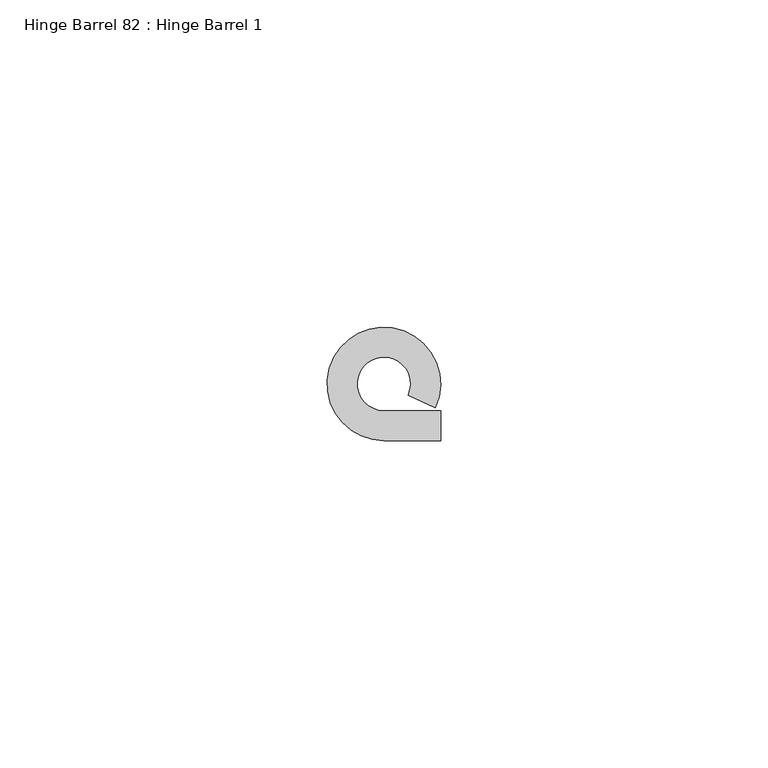
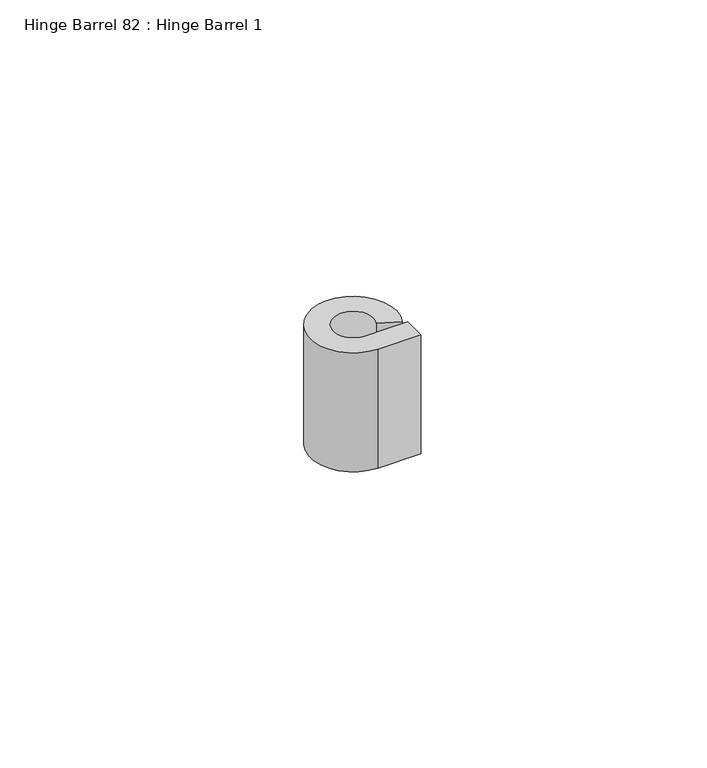
"""IFC4 building model written with IfcOpenShell, lengths in millimetres: proxy geometry, Hinge Barrel 82 : Hinge Barrel 1."""

from ifc_helpers import new_model, si_unit, point, frame, frame_2d, origin, place, context, project, spatial, polyline, circle_curve, trimmed, segment, composite_curve, outline, extrude, source, transform, mapped, element, save


def hinge_barrel_82_hinge_barrel_1_181395a2(model_context):
    return source(origin(), model_context, "Body", "SweptSolid", [
        extrude(outline(composite_curve([segment(polyline([(587323.2214739, -531780.6943841), (587327.7934739, -531780.6943841), (587327.7934739, -531785.2584466), (587319.1320739, -531785.2584466)]), True, "CONTINUOUS"), segment(trimmed(circle_curve(frame_2d((587319.1320739, -531776.6049841)), 8.6534625), [point((587319.1320739, -531785.2584466))], [point((587326.986084, -531780.2377433))], False, "CARTESIAN"), True, "CONTINUOUS"), segment(polyline([(587326.986084, -531780.2377433), (587322.8436736, -531778.321731)]), True, "CONTINUOUS"), segment(trimmed(circle_curve(frame_2d((587319.1320739, -531776.6049841)), 4.0894), [point((587322.8436736, -531778.321731))], [point((587319.1320739, -531780.6943841))], True, "CARTESIAN"), True, "CONTINUOUS"), segment(polyline([(587319.1320739, -531780.6943841), (587323.2214739, -531780.6943841)]), True, "CONTINUOUS")], self_intersect=False)), frame((0.0, 0.0, 2038.35), z_axis=(0.0, 0.0, 1.0), x_axis=(1.0, 0.0, 0.0)), (0.0, 0.0, 1.0), 25.4),
    ])


if __name__ == "__main__":
    model = new_model("IFC4")
    model_context = context("Model", 3, world=origin())
    ifc_project = project(units=[si_unit("LENGTHUNIT", "METRE", prefix="MILLI")], contexts=[model_context])
    site = spatial("IfcSite", under=ifc_project)
    building = spatial("IfcBuilding", under=site)
    placement = place(None, origin())
    hinge_barrel_82_hinge_barrel_1_shape = hinge_barrel_82_hinge_barrel_1_181395a2(model_context)
    element("IfcBuildingElementProxy", 1, Name="Hinge Barrel 82 : Hinge Barrel 1", ObjectType="Hinge Barrel 82 : Hinge Barrel 1", at=placement, inside=building, context=model_context, shape_type="MappedRepresentation", body=[
        mapped(hinge_barrel_82_hinge_barrel_1_shape, transform((0.0, 0.0, 0.0), x_axis=(1.0, 0.0, 0.0), y_axis=(0.0, 1.0, 0.0), z_axis=(0.0, 0.0, 1.0))),
    ])
    save(model, "model.ifc")

# Revit data of these elements
# Element 1 (IfcBuildingElementProxy, "Hinge Barrel 82 : Hinge Barrel 1")
#   Materials on its faces: "6\"X6\" WELD-ON STL BUTT HINGE"
# Materials
#   "6\"X6\" WELD-ON STL BUTT HINGE": class "Metal", colour RGB 189 187 185, transparency 0, Description = "Carbon steel", Cost = 0
